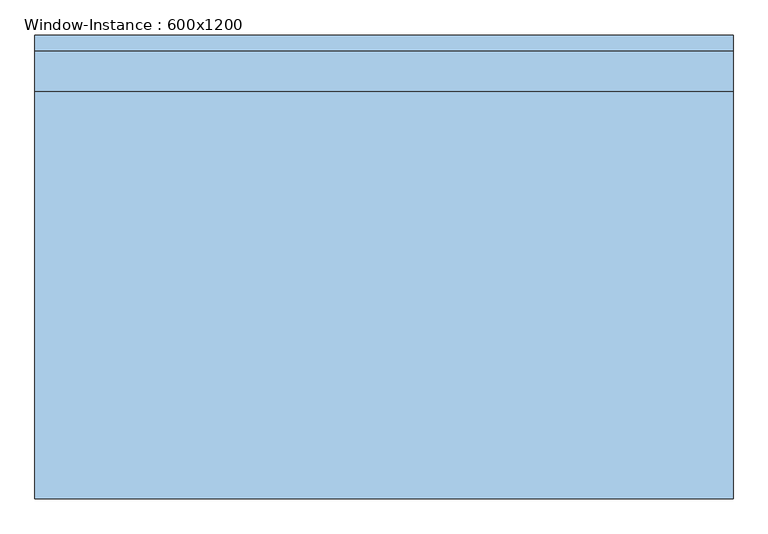
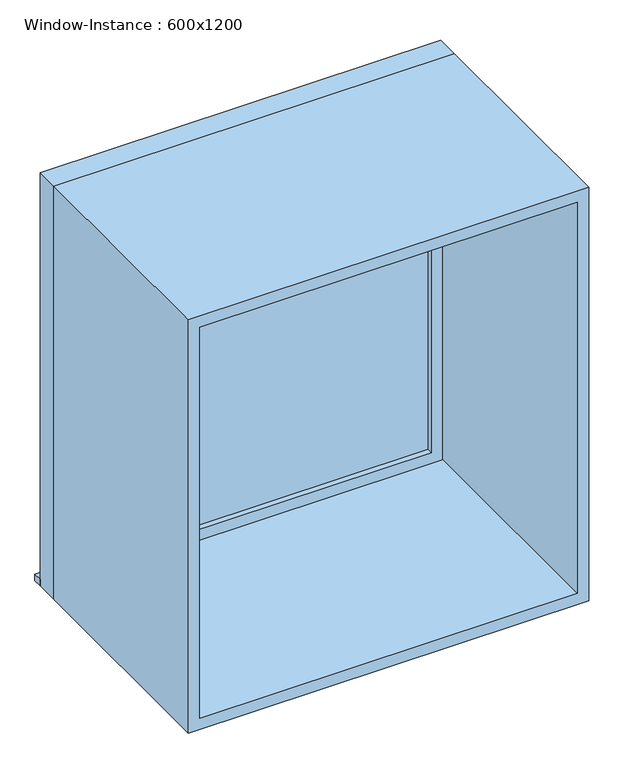
"""IFC4 building model written with IfcOpenShell, lengths in millimetres: window geometry, Window-Instance : 600x1200."""

from ifc_helpers import new_model, si_unit, frame, origin, place, context, project, spatial, polyline, outline, extrude, source, transform, mapped, element, save


def window_instance_600x1200_58ea7eaf(model_context):
    return source(origin(), model_context, "Body", "SweptSolid", [
        extrude(outline(polyline([(-588.1, 377.9), (511.9, 377.9), (511.9, 352.5), (-588.1, 352.5), (-588.1, 377.9)])), frame((0.0, 0.0, 900.0), z_axis=(0.0, 0.0, 1.0), x_axis=(1.0, 0.0, 0.0)), (0.0, 0.0, 1.0), 19.05),
        extrude(outline(polyline([(448.4, 303.925), (-524.6, 303.925), (-524.6, 316.625), (448.4, 316.625), (448.4, 303.925)])), frame((0.0, 0.0, 963.5), z_axis=(0.0, 0.0, 1.0), x_axis=(1.0, 0.0, 0.0)), (0.0, 0.0, 1.0), 1073.0),
        extrude(outline(polyline([(2080.95, -569.05), (919.05, -569.05), (919.05, 492.85), (2080.95, 492.85), (2080.95, -569.05)]), holes=[polyline([(2036.5, -524.6), (2036.5, 448.4), (963.5, 448.4), (963.5, -524.6), (2036.5, -524.6)])]), frame((0.0, 288.05, 0.0), z_axis=(0.0, 1.0, 0.0), x_axis=(0.0, 0.0, 1.0)), (0.0, 0.0, 1.0), 44.45),
        extrude(outline(polyline([(2100.0, -588.1), (900.0, -588.1), (900.0, 511.9), (2100.0, 511.9), (2100.0, -588.1)]), holes=[polyline([(2068.25, -556.35), (2068.25, 480.15), (931.75, 480.15), (931.75, -556.35), (2068.25, -556.35)])]), frame((0.0, -352.5, 0.0), z_axis=(0.0, 1.0, 0.0), x_axis=(0.0, 0.0, 1.0)), (0.0, 0.0, 1.0), 640.55),
        extrude(outline(polyline([(2100.0, 511.9), (2100.0, -588.1), (900.0, -588.1), (900.0, 511.9), (2100.0, 511.9)]), holes=[polyline([(2080.95, 492.85), (919.05, 492.85), (919.05, -569.05), (2080.95, -569.05), (2080.95, 492.85)])]), frame((0.0, 288.05, 0.0), z_axis=(0.0, 1.0, 0.0), x_axis=(0.0, 0.0, 1.0)), (0.0, 0.0, 1.0), 64.45),
    ])


if __name__ == "__main__":
    model = new_model("IFC4")
    model_context = context("Model", 3, world=origin())
    ifc_project = project(units=[si_unit("LENGTHUNIT", "METRE", prefix="MILLI")], contexts=[model_context])
    site = spatial("IfcSite", under=ifc_project)
    building = spatial("IfcBuilding", under=site)
    placement = place(None, origin())
    window_instance_600x1200_shape = window_instance_600x1200_58ea7eaf(model_context)
    element("IfcWindow", 1, ObjectType="Window-Instance : 600x1200", at=placement, inside=building, context=model_context, shape_type="MappedRepresentation", body=[
        mapped(window_instance_600x1200_shape, transform((0.0, 0.0, 0.0), x_axis=(1.0, 0.0, 0.0), y_axis=(0.0, 1.0, 0.0), z_axis=(0.0, 0.0, 1.0))),
    ])
    save(model, "model.ifc")

# Revit data of these elements
# Type "Window-Instance : 600x1200"
#   Type Mark = "7"
#   Construction Type Id = "GSP4R"
#   Assembly Code = "B2020100"
#   Analytic Construction = "1/8 in Pilkington single glazing"
#   Visual Light Transmittance = 0.9
#   Thermal Resistance (R) = 0.149095 (m²·K)/W
#   Solar Heat Gain Coefficient = 0.86
#   Heat Transfer Coefficient (U) = 6.70716 W/(m²·K)
#   Height [instance default] = 1200 mm
#   Default Sill Height = 900 mm
#   Width [instance default] = 600 mm
#   Window Inset = 20 mm
#   Glass Pane Material = WW-EC-GL-Storefront
#   Sash Material = WW-EC-RGB-White
#   Wall Closure = (empty or 0)
# Element 1 (IfcWindow, "Window-Instance : 600x1200")
#   Width = 1100 mm
#   Materials on its faces: "WW-EC-RGB-White", "WW-EC-GL-Storefront"
# Materials
#   "WW-EC-GL-Storefront": class "Glass", colour RGB 236 240 239, transparency 0.85, Description = "Storefront Glass", Cost = 0
#   "WW-EC-RGB-White": class "Generic", colour RGB 255 255 255, transparency 0, Comments = "If region requests off-white, swith asset color to RGB 231-228-220", Description = "Generic Color", Cost = 0
